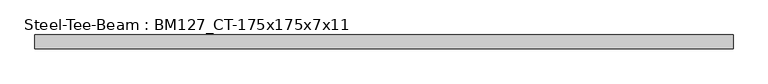
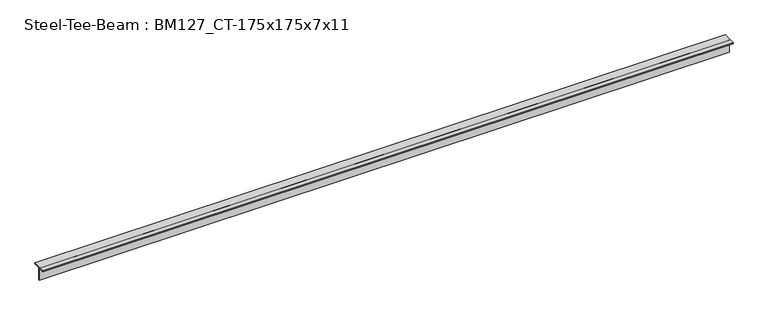
"""IFC4 building model written with IfcOpenShell, lengths in millimetres: beam geometry, Steel-Tee-Beam : BM127_CT-175x175x7x11."""

import ifcopenshell
import ifcopenshell.guid

model = None  # the IFC model being written
_history = None  # IfcOwnerHistory: only IFC2X3 demands one
_inside = {}  # id of a spatial element -> (the spatial element, [elements in it])
_under = {}  # id of a project, library or spatial element -> (it, [spatial elements below it])
_declared = {}  # id of a project -> (the project, [libraries it declares])
_typed = {}  # id of a type object -> (the type object, [elements of that type])
_made_of = {}  # id of a material, layer set ... -> (it, [elements and type objects made of it])


def new_model(schema):
    """Start an empty IFC model of exactly this schema.

    Asked for "IFC4X3", IfcOpenShell would pick the latest addendum, in which some entities
    have other attributes; the version numbers below select the first issue.
    IFC2X3 requires an IfcOwnerHistory on every rooted entity: one is made here for all.
    """
    global model, _history
    if schema == "IFC4X3":
        model = ifcopenshell.file(schema_version=(4, 3, 0, 0))
    else:
        model = ifcopenshell.file(schema=schema)
    _inside.clear()
    _under.clear()
    _declared.clear()
    _typed.clear()
    _made_of.clear()
    _history = None
    if model.schema == "IFC2X3":
        org = make("IfcOrganization", Name="unknown")
        user = make(
            "IfcPersonAndOrganization",
            ThePerson=make("IfcPerson", FamilyName="unknown"),
            TheOrganization=org,
        )
        app = make(
            "IfcApplication",
            ApplicationDeveloper=org,
            Version="unknown",
            ApplicationFullName="unknown",
            ApplicationIdentifier="unknown",
        )
        _history = make(
            "IfcOwnerHistory",
            OwningUser=user,
            OwningApplication=app,
            ChangeAction="ADDED",
            CreationDate=0,
        )
    return model


def make(cls, **values):
    """One entity of the class cls with the attributes given. An attribute that is None is left unset."""
    return model.create_entity(
        cls, **{name: value for name, value in values.items() if value is not None}
    )


def rooted(cls, **values):
    """An entity with a GlobalId (a new one), such as an element, a storey or a relation."""
    return make(cls, GlobalId=ifcopenshell.guid.new(), OwnerHistory=_history, **values)


def si_unit(unit_type, name, prefix=None):
    """IfcSIUnit, for example si_unit("LENGTHUNIT", "METRE", prefix="MILLI")."""
    return make("IfcSIUnit", UnitType=unit_type, Prefix=prefix, Name=name)


def assignment(units):
    """IfcUnitAssignment: the units of a project."""
    return None if units is None else make("IfcUnitAssignment", Units=units)


def point(xyz):
    """IfcCartesianPoint."""
    return None if xyz is None else make("IfcCartesianPoint", Coordinates=xyz)


def direction(xyz):
    """IfcDirection."""
    return None if xyz is None else make("IfcDirection", DirectionRatios=xyz)


def frame(location, z_axis=None, x_axis=None):
    """IfcAxis2Placement3D, a coordinate frame: its origin and axes. An axis left out is left unset."""
    return make(
        "IfcAxis2Placement3D",
        Location=point(location),
        Axis=direction(z_axis),
        RefDirection=direction(x_axis),
    )


def frame_2d(location, x_axis=None):
    """IfcAxis2Placement2D, a coordinate frame in the plane: its origin and x axis."""
    return make(
        "IfcAxis2Placement2D", Location=point(location), RefDirection=direction(x_axis)
    )


def origin():
    """The frame at (0, 0, 0) with its axes left unset."""
    return frame((0.0, 0.0, 0.0))


def place(relative_to, where):
    """IfcLocalPlacement: puts the frame where relative to a parent placement (None: the world)."""
    return make(
        "IfcLocalPlacement", PlacementRelTo=relative_to, RelativePlacement=where
    )


def context(
    kind, dimensions, precision=None, world=None, true_north=None, identifier=None
):
    """IfcGeometricRepresentationContext, for example the 3D "Model" context."""
    return make(
        "IfcGeometricRepresentationContext",
        ContextIdentifier=identifier,
        ContextType=kind,
        CoordinateSpaceDimension=dimensions,
        Precision=precision,
        WorldCoordinateSystem=world,
        TrueNorth=true_north,
    )


def project(units=None, contexts=None):
    """IfcProject with its units and contexts."""
    return rooted(
        "IfcProject",
        Name="project",
        RepresentationContexts=contexts,
        UnitsInContext=assignment(units),
    )


def spatial(cls, under=None, at=None, **own):
    """A site, building, storey or space (cls), placed at a placement, below another one or the project."""
    s = rooted(cls, ObjectPlacement=at, **own)
    if under is not None:
        _under.setdefault(under.id(), (under, []))[1].append(s)
    return s


def polyline(points):
    """IfcPolyline through the points."""
    return make("IfcPolyline", Points=[point(p) for p in points])


def circle_curve(where, radius):
    """IfcCircle in the frame where."""
    return make("IfcCircle", Position=where, Radius=radius)


def trimmed(basis, trim1, trim2, sense, master):
    """IfcTrimmedCurve: the piece of a basis curve between two trims."""
    return make(
        "IfcTrimmedCurve",
        BasisCurve=basis,
        Trim1=trim1,
        Trim2=trim2,
        SenseAgreement=sense,
        MasterRepresentation=master,
    )


def segment(curve, same_sense, transition):
    """IfcCompositeCurveSegment."""
    return make(
        "IfcCompositeCurveSegment",
        Transition=transition,
        SameSense=same_sense,
        ParentCurve=curve,
    )


def composite_curve(segments, self_intersect=None):
    """IfcCompositeCurve: segments joined end to end."""
    return make("IfcCompositeCurve", Segments=segments, SelfIntersect=self_intersect)


def outline(outer, holes=None, kind="AREA"):
    """IfcArbitraryClosedProfileDef: a profile drawn as a closed curve; with holes, ...WithVoids."""
    if holes is None:
        return make("IfcArbitraryClosedProfileDef", ProfileType=kind, OuterCurve=outer)
    return make(
        "IfcArbitraryProfileDefWithVoids",
        ProfileType=kind,
        OuterCurve=outer,
        InnerCurves=holes,
    )


def extrude(swept, where, along, depth):
    """IfcExtrudedAreaSolid: the profile swept, set in the frame where, extruded along a direction by depth."""
    return make(
        "IfcExtrudedAreaSolid",
        SweptArea=swept,
        Position=where,
        ExtrudedDirection=direction(along),
        Depth=depth,
    )


def shape(context_of_items, identifier, shape_type, items):
    """IfcShapeRepresentation: the items that make up one representation, for example the "Body"."""
    return make(
        "IfcShapeRepresentation",
        ContextOfItems=context_of_items,
        RepresentationIdentifier=identifier,
        RepresentationType=shape_type,
        Items=items,
    )


def source(mapping_origin, context_of_items, identifier, shape_type, items):
    """IfcRepresentationMap: a shape defined once, which mapped items show again and again."""
    return make(
        "IfcRepresentationMap",
        MappingOrigin=mapping_origin,
        MappedRepresentation=shape(context_of_items, identifier, shape_type, items),
    )


def transform(
    local_origin,
    x_axis=None,
    y_axis=None,
    z_axis=None,
    scale=None,
    scale2=None,
    scale3=None,
    uniform=True,
):
    """IfcCartesianTransformationOperator3D, or its non-uniform kind. x_axis, y_axis, z_axis: its Axis1, 2, 3."""
    if uniform:
        return make(
            "IfcCartesianTransformationOperator3D",
            Axis1=direction(x_axis),
            Axis2=direction(y_axis),
            LocalOrigin=point(local_origin),
            Scale=scale,
            Axis3=direction(z_axis),
        )
    return make(
        "IfcCartesianTransformationOperator3DnonUniform",
        Axis1=direction(x_axis),
        Axis2=direction(y_axis),
        LocalOrigin=point(local_origin),
        Scale=scale,
        Axis3=direction(z_axis),
        Scale2=scale2,
        Scale3=scale3,
    )


def mapped(mapping_source, mapping_target):
    """IfcMappedItem: shows the shape of a source again, moved by a transform."""
    return make(
        "IfcMappedItem", MappingSource=mapping_source, MappingTarget=mapping_target
    )


def made_of(thing, what):
    """Note that an element or type object is made of a material, layer set ...; save() writes the relation."""
    if what is not None:
        _made_of.setdefault(what.id(), (what, []))[1].append(thing)
    return thing


def element(
    cls,
    number,
    at=None,
    inside=None,
    cuts=None,
    type_object=None,
    material=None,
    context=None,
    identifier="Body",
    shape_type=None,
    held_by="IfcProductDefinitionShape",
    body=None,
    shapes=None,
    **own,
):
    """One element of the class cls, such as IfcWall. Its Tag is "e" and its number.

    at: its placement. inside: the storey or other place that contains it. cuts: it is an
    opening in that element (IfcRelVoidsElement). A single representation is given by context,
    identifier, shape_type and body (its items); several are given by shapes. held_by: the class
    of the entity that holds the representations. save() writes the other relations.
    """
    e = rooted(cls, Tag="e%d" % number, ObjectPlacement=at, **own)
    if body is not None:
        shapes = [shape(context, identifier, shape_type, body)]
    if shapes is not None:
        e.Representation = make(held_by, Representations=shapes)
    if inside is not None:
        _inside.setdefault(inside.id(), (inside, []))[1].append(e)
    if cuts is not None:
        rooted(
            "IfcRelVoidsElement", RelatingBuildingElement=cuts, RelatedOpeningElement=e
        )
    if type_object is not None:
        _typed.setdefault(type_object.id(), (type_object, []))[1].append(e)
    return made_of(e, material)


def aggregate(whole, parts):
    """IfcRelAggregates: a whole, such as a stair, and the parts it consists of."""
    return rooted("IfcRelAggregates", RelatingObject=whole, RelatedObjects=parts)


def save(model, path):
    """Write the relations noted so far, then the file.

    IfcRelAggregates (storeys below a building ...), IfcRelContainedInSpatialStructure (elements
    in a storey), IfcRelDefinesByType, IfcRelAssociatesMaterial and IfcRelDeclares: one each for
    every whole, place, type object, material and project.
    """
    for whole, parts in _under.values():
        aggregate(whole, parts)
    for where, things in _inside.values():
        rooted(
            "IfcRelContainedInSpatialStructure",
            RelatedElements=things,
            RelatingStructure=where,
        )
    for kind, things in _typed.values():
        rooted("IfcRelDefinesByType", RelatedObjects=things, RelatingType=kind)
    for what, things in _made_of.values():
        rooted("IfcRelAssociatesMaterial", RelatedObjects=things, RelatingMaterial=what)
    for by, libraries in _declared.values():
        rooted("IfcRelDeclares", RelatingContext=by, RelatedDefinitions=libraries)
    model.write(path)


def steel_tee_beam_bm127_ct_175x175x7x11_3d5bc00e(model_context):
    return source(origin(), model_context, "Body", "SweptSolid", [
        extrude(outline(composite_curve([segment(polyline([(87.5, 87.5), (87.5, 76.5), (17.5, 76.5)]), True, "CONTINUOUS"), segment(trimmed(circle_curve(frame_2d((17.5, 62.5)), 14.0), [point((17.5, 76.5))], [point((3.5, 62.5))], True, "CARTESIAN"), True, "CONTINUOUS"), segment(polyline([(3.5, 62.5), (3.5, -87.5), (-3.5, -87.5), (-3.5, 62.5)]), True, "CONTINUOUS"), segment(trimmed(circle_curve(frame_2d((-17.5, 62.5)), 14.0), [point((-3.5, 62.5))], [point((-17.5, 76.5))], True, "CARTESIAN"), True, "CONTINUOUS"), segment(polyline([(-17.5, 76.5), (-87.5, 76.5), (-87.5, 87.5), (87.5, 87.5)]), True, "CONTINUOUS")], self_intersect=False)), frame((-4298.1792655, 0.0, 0.0), z_axis=(1.0, 0.0, 0.0), x_axis=(0.0, 1.0, 0.0)), (0.0, 0.0, 1.0), 8725.555017),
    ])


if __name__ == "__main__":
    model = new_model("IFC4")
    model_context = context("Model", 3, world=origin())
    ifc_project = project(units=[si_unit("LENGTHUNIT", "METRE", prefix="MILLI")], contexts=[model_context])
    site = spatial("IfcSite", under=ifc_project)
    building = spatial("IfcBuilding", under=site)
    placement = place(None, origin())
    steel_tee_beam_bm127_ct_175x175x7x11_shape = steel_tee_beam_bm127_ct_175x175x7x11_3d5bc00e(model_context)
    element("IfcBeam", 1, ObjectType="Steel-Tee-Beam : BM127_CT-175x175x7x11", at=placement, inside=building, context=model_context, shape_type="MappedRepresentation", body=[
        mapped(steel_tee_beam_bm127_ct_175x175x7x11_shape, transform((0.0, 0.0, 0.0), x_axis=(1.0, 0.0, 0.0), y_axis=(0.0, 1.0, 0.0), z_axis=(0.0, 0.0, 1.0))),
    ])
    save(model, "model.ifc")

# Revit data of these elements
# Type "Steel-Tee-Beam : BM127_CT-175x175x7x11"
#   Surface Area = 0.00 m²/m
#   Section Area = 31.57 cm²
#   Mass per Unit Length = 24.80 kg/m
#   Length [instance default] = 1524 mm
#   bf = 175 mm
#   d = 175 mm
#   k = 25 mm
#   kr = 14 mm
#   tf = 11 mm
#   tw = 7 mm
#   hec_material4 [instance default] = none
#   hec_material3 [instance default] = none
#   hec_material2 [instance default] = none
#   hec_material1 [instance default] = none
#   Structural Material [instance default] = Steel, 45-345
#   Assembly Code = ""
# Element 1 (IfcBeam, "Steel-Tee-Beam : BM127_CT-175x175x7x11")
#   hec_material3 = F01AC000-00002_Building/Shelter Fire Proofing Work_Intumescent Coating Type_1 hr. rating (UL 1709))
#   hec_material2 = S01AA010-00002_Main Steel Structure Fabrication Work_Shelter/Building_Steel Painting/Coating_for Fireproofed Steel Surface, Surface Preparation & Primer Coat
#   hec_material1 = S03AA029-00001_Main Steel Structure Erection Work_Shelter/Building_Light Steel
#   Structural Material = S01AA003-00001_Main Steel Structure Fabrication Work_Shelter/Building_Light Steel - Standard
#   Materials on its faces: "S01AA003-00001_Main Steel Structure Fabrication Work_Shelter/Building_Light Steel - Standard"
# Materials
#   "Steel, 45-345": class "Metal", colour RGB 189 187 185, transparency 0, Description = "Steel 345 MPa", Cost = 0
#   "S01AA003-00001_Main Steel Structure Fabrication Work_Shelter/Building_Light Steel - Standard": class "Metal", colour RGB 120 120 120, transparency 0, Comments = "(30KG/M>Weight)", Description = "Structural steel 50ksi", W00) Work Master Code = "S01AA003-00001", W01) Work Master_Lv1 = "Main Steel Structure Fabrication Work", W02) Work Master_Lv2 = "Shelter/Building", W03) Work Master_Spec.1 = "Light Steel - Standard (30KG/M>Weight)", Cost = 0
#   "F01AC000-00002_Building/Shelter Fire Proofing Work_Intumescent Coating Type_1 hr. rating (UL 1709))": class "Metal", colour RGB 255 128 128, transparency 0, Description = "Paint finished steel", W00) Work Master Code = "F01AC000-00002", W01) Work Master_Lv1 = "Building/Shelter Fire Proofing Work", W02) Work Master_Lv2 = "Intumescent Coating Type", W03) Work Master_Spec.1 = "1 hr. rating (UL 1709)", Cost = 0
#   "S01AA010-00002_Main Steel Structure Fabrication Work_Shelter/Building_Steel Painting/Coating_for Fireproofed Steel Surface, Surface Preparation & Primer Coat": class "Metal", colour RGB 120 120 120, transparency 0, Description = "Paint finished steel", W00) Work Master Code = "SS01AA010-00002", W01) Work Master_Lv1 = "Main Steel Structure Fabrication Work", W02) Work Master_Lv2 = "Shelter/Building", W03) Work Master_Spec.1 = "Steel Painting/Coating", W04) Work Master_Spec.2 = "for Fireproofed Steel Surface, Surface Preparation & Primer Coat", Cost = 0
#   "S03AA029-00001_Main Steel Structure Erection Work_Shelter/Building_Light Steel": class "Metal", colour RGB 120 120 120, transparency 0, Comments = "(30KG/M>Weight)", Description = "Structural steel 50ksi", W00) Work Master Code = "S03AA029-00001", W01) Work Master_Lv1 = "Main Steel Structure Erection Work", W02) Work Master_Lv2 = "Shelter/Building", W03) Work Master_Spec.1 = "Light Steel (30KG/M>Weight)", Cost = 0
